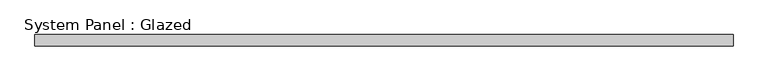
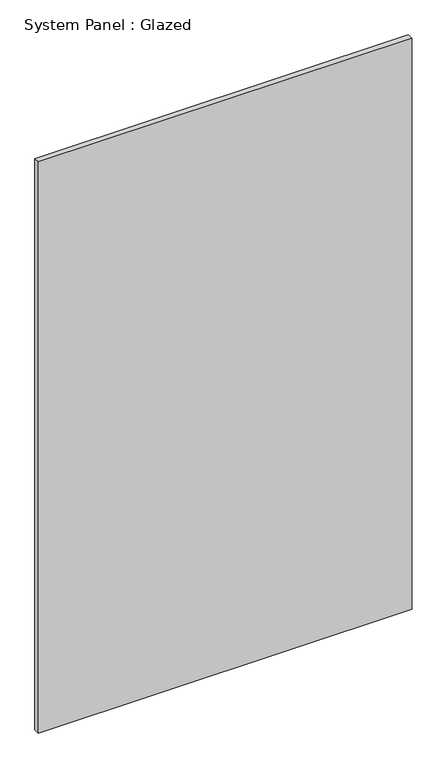
"""IFC4 building model written with IfcOpenShell, lengths in millimetres: plate geometry, System Panel : Glazed."""

from ifc_helpers import new_model, si_unit, origin, origin_with_axes, place, context, project, spatial, polyline, outline, extrude, source, transform, mapped, element, save


def system_panel_glazed_52effc56(model_context):
    return source(origin(), model_context, "Body", "SweptSolid", [
        extrude(outline(polyline([(796.9250048, 19.05), (-796.9250048, 19.05), (-796.9250048, 44.45), (796.9250048, 44.45), (796.9250048, 19.05)])), origin_with_axes(), (0.0, 0.0, 1.0), 2578.1),
    ])


if __name__ == "__main__":
    model = new_model("IFC4")
    model_context = context("Model", 3, world=origin())
    ifc_project = project(units=[si_unit("LENGTHUNIT", "METRE", prefix="MILLI")], contexts=[model_context])
    site = spatial("IfcSite", under=ifc_project)
    building = spatial("IfcBuilding", under=site)
    placement = place(None, origin())
    system_panel_glazed_shape = system_panel_glazed_52effc56(model_context)
    element("IfcPlate", 1, ObjectType="System Panel : Glazed", at=placement, inside=building, context=model_context, shape_type="MappedRepresentation", body=[
        mapped(system_panel_glazed_shape, transform((0.0, 0.0, 0.0), x_axis=(1.0, 0.0, 0.0), y_axis=(0.0, 1.0, 0.0), z_axis=(0.0, 0.0, 1.0))),
    ])
    save(model, "model.ifc")

# Revit data of these elements
# Type "System Panel : Glazed"
#   Construction Type Id = "GSP4R"
#   Analytic Construction = "1/8 in Pilkington single glazing"
#   Visual Light Transmittance = 0.9
#   Solar Heat Gain Coefficient = 0.86
#   Heat Transfer Coefficient (U) = 1.18115 BTU/(h·ft²·°F)
#   Define Thermal Properties by = 1
# Element 1 (IfcPlate, "System Panel : Glazed")
#   Materials on its faces: "Glass"
# Materials
#   "Glass": class "Glass", colour RGB 0 128 192, transparency 0.75, Description = "Soda Lime Glass", Cost = 0
